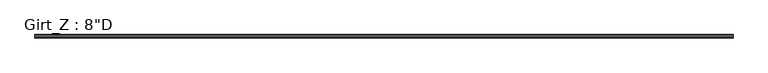
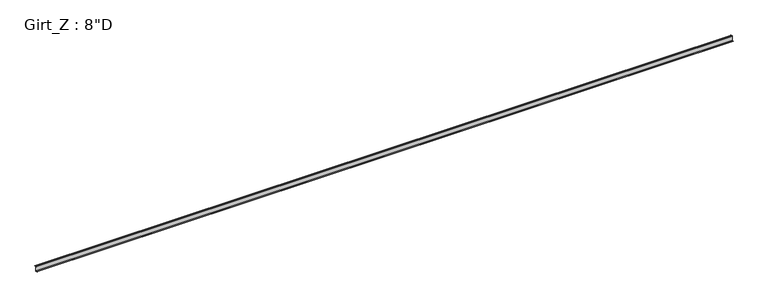
"""IFC4 building model written with IfcOpenShell, lengths in millimetres: beam geometry."""

from ifc_helpers import new_model, si_unit, point, frame, frame_2d, origin, place, context, project, spatial, polyline, circle_curve, trimmed, segment, composite_curve, outline, extrude, source, transform, mapped, element, save


def beam_1d69901f(model_context):
    return source(origin(), model_context, "Body", "SweptSolid", [
        extrude(outline(composite_curve([segment(polyline([(63.5, 101.6), (75.745104, 87.0068534), (73.6169367, 85.221109), (62.204539, 98.821875), (3.3005807, 98.821875)]), True, "CONTINUOUS"), segment(trimmed(circle_curve(frame_2d((3.3741066, 96.8381931)), 1.9850441), [point((3.3005807, 98.821875))], [point((1.3890625, 96.8381931))], True, "CARTESIAN"), True, "CONTINUOUS"), segment(polyline([(1.3890625, 96.8381931), (1.3890625, -96.8375)]), True, "CONTINUOUS"), segment(trimmed(circle_curve(frame_2d((-3.3734375, -96.8375)), 4.7625), [point((1.3890625, -96.8375))], [point((-3.3734375, -101.6))], False, "CARTESIAN"), True, "CONTINUOUS"), segment(polyline([(-3.3734375, -101.6), (-63.5, -101.6), (-75.745104, -87.0068534), (-73.6169367, -85.221109), (-62.204539, -98.821875), (-3.2694106, -98.821875)]), True, "CONTINUOUS"), segment(trimmed(circle_curve(frame_2d((-3.3748024, -96.8389339)), 1.9857399), [point((-3.2694106, -98.821875))], [point((-1.3890625, -96.8389339))], True, "CARTESIAN"), True, "CONTINUOUS"), segment(polyline([(-1.3890625, -96.8389339), (-1.3890625, 96.8375)]), True, "CONTINUOUS"), segment(trimmed(circle_curve(frame_2d((3.3734375, 96.8375)), 4.7625), [point((-1.3890625, 96.8375))], [point((3.3734375, 101.6))], False, "CARTESIAN"), True, "CONTINUOUS"), segment(polyline([(3.3734375, 101.6), (63.5, 101.6)]), True, "CONTINUOUS")], self_intersect=False)), frame((-15307.7423336, 0.0, 0.0), z_axis=(1.0, 0.0, 0.0), x_axis=(0.0, 1.0, 0.0)), (0.0, 0.0, 1.0), 29718.7823803),
    ])


if __name__ == "__main__":
    model = new_model("IFC4")
    model_context = context("Model", 3, world=origin())
    ifc_project = project(units=[si_unit("LENGTHUNIT", "METRE", prefix="MILLI")], contexts=[model_context])
    site = spatial("IfcSite", under=ifc_project)
    building = spatial("IfcBuilding", under=site)
    placement = place(None, origin())
    beam_shape = beam_1d69901f(model_context)
    element("IfcBeam", 1, ObjectType="Girt_Z : 8\"D", at=placement, inside=building, context=model_context, shape_type="MappedRepresentation", body=[
        mapped(beam_shape, transform((0.0, 0.0, 0.0), x_axis=(1.0, 0.0, 0.0), y_axis=(0.0, 1.0, 0.0), z_axis=(0.0, 0.0, 1.0))),
    ])
    save(model, "model.ifc")

# Revit data of these elements
# Type "Girt_Z : 8\"D"
#   Web_Thickness = 0' - 0 7/64"
#   Length [instance default] = 10' - 0"
#   Leg_1 = 0' - 2 1/2"
#   Height = 0' - 8"
#   Structural Material [instance default] = none
# Element 1 (IfcBeam, "Girt_Z : 8\"D")
#   Structural Material = Steel
#   Materials on its faces: "Steel"
# Materials
#   "Steel": class "Metal", colour RGB 118 118 114, transparency 0, Description = "Steel, mill finish", Cost = 0
